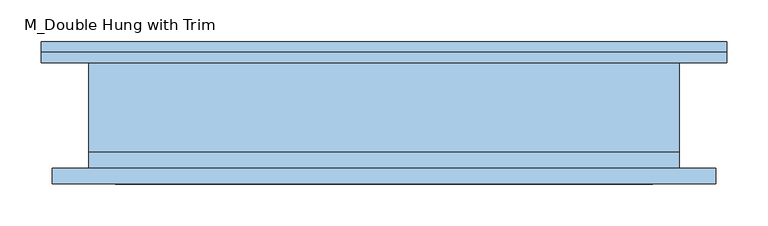
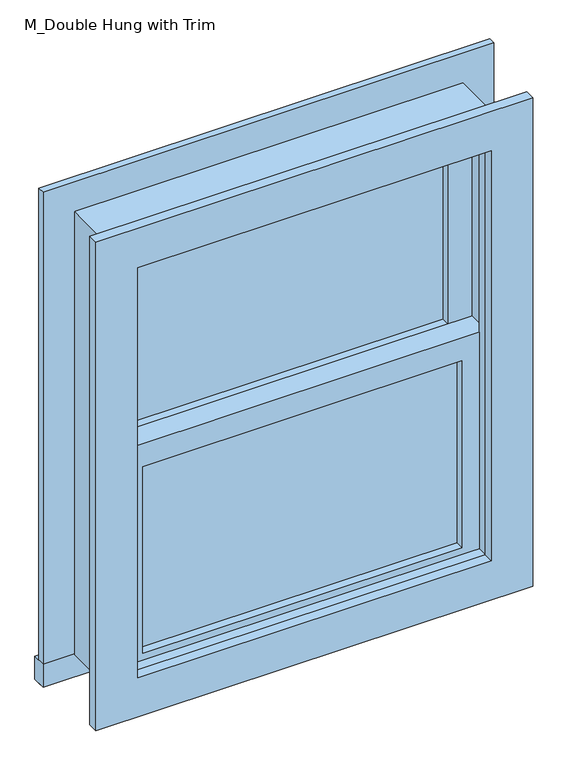
"""IFC4 building model written with IfcOpenShell, lengths in millimetres: window geometry, M_Double Hung with Trim."""

from ifc_helpers import new_model, si_unit, frame, origin, place, context, project, spatial, polyline, outline, extrude, source, transform, mapped, element, save


def m_double_hung_with_trim_a11a7e0a(model_context):
    return source(origin(), model_context, "Body", "SweptSolid", [
        extrude(outline(polyline([(-292.1, -15.825), (292.1, -15.825), (292.1, -28.525), (-292.1, -28.525), (-292.1, -15.825)])), frame((0.0, 0.0, 628.65), z_axis=(0.0, 0.0, 1.0), x_axis=(1.0, 0.0, 0.0)), (0.0, 0.0, 1.0), 361.95),
        extrude(outline(polyline([(1035.05, -336.55), (584.2, -336.55), (584.2, 336.55), (1035.05, 336.55), (1035.05, -336.55)]), holes=[polyline([(990.6, -292.1), (990.6, 292.1), (628.65, 292.1), (628.65, -292.1), (990.6, -292.1)])]), frame((0.0, -44.4, 0.0), z_axis=(0.0, 1.0, 0.0), x_axis=(0.0, 0.0, 1.0)), (0.0, 0.0, 1.0), 44.45),
        extrude(outline(polyline([(-412.75, 89.2), (412.75, 89.2), (412.75, 63.5), (-412.75, 63.5), (-412.75, 89.2)])), frame((0.0, 0.0, 539.75), z_axis=(0.0, 0.0, 1.0), x_axis=(1.0, 0.0, 0.0)), (0.0, 0.0, 1.0), 44.45),
        extrude(outline(polyline([(1498.6, -412.75), (539.75, -412.75), (539.75, 412.75), (1498.6, 412.75), (1498.6, -412.75)]), holes=[polyline([(1422.4, -336.55), (1422.4, 336.55), (584.2, 336.55), (584.2, -336.55), (1422.4, -336.55)])]), frame((0.0, 63.5, 0.0), z_axis=(0.0, 1.0, 0.0), x_axis=(0.0, 0.0, 1.0)), (0.0, 0.0, 1.0), 13.0),
        extrude(outline(polyline([(1485.9, 400.05), (1485.9, -400.05), (539.75, -400.05), (539.75, 400.05), (1485.9, 400.05)]), holes=[polyline([(1409.7, 323.85), (615.95, 323.85), (615.95, -323.85), (1409.7, -323.85), (1409.7, 323.85)])]), frame((0.0, -82.5, 0.0), z_axis=(0.0, 1.0, 0.0), x_axis=(0.0, 0.0, 1.0)), (0.0, 0.0, 1.0), 19.0),
        extrude(outline(polyline([(292.1, 15.925), (-292.1, 15.925), (-292.1, 28.625), (292.1, 28.625), (292.1, 15.925)])), frame((0.0, 0.0, 1035.05), z_axis=(0.0, 0.0, 1.0), x_axis=(1.0, 0.0, 0.0)), (0.0, 0.0, 1.0), 342.9),
        extrude(outline(polyline([(1422.4, -336.55), (990.6, -336.55), (990.6, 336.55), (1422.4, 336.55), (1422.4, -336.55)]), holes=[polyline([(1377.95, -292.1), (1377.95, 292.1), (1035.05, 292.1), (1035.05, -292.1), (1377.95, -292.1)])]), frame((0.0, 0.05, 0.0), z_axis=(0.0, 1.0, 0.0), x_axis=(0.0, 0.0, 1.0)), (0.0, 0.0, 1.0), 44.45),
        extrude(outline(polyline([(1441.45, -355.6), (584.2, -355.6), (584.2, 355.6), (1441.45, 355.6), (1441.45, -355.6)]), holes=[polyline([(1409.7, -323.85), (1409.7, 323.85), (615.95, 323.85), (615.95, -323.85), (1409.7, -323.85)])]), frame((0.0, -63.5, 0.0), z_axis=(0.0, 1.0, 0.0), x_axis=(0.0, 0.0, 1.0)), (0.0, 0.0, 1.0), 19.1),
        extrude(outline(polyline([(1441.45, 355.6), (1441.45, -355.6), (584.2, -355.6), (584.2, 355.6), (1441.45, 355.6)]), holes=[polyline([(1422.4, 336.55), (603.25, 336.55), (603.25, -336.55), (1422.4, -336.55), (1422.4, 336.55)])]), frame((0.0, -44.4, 0.0), z_axis=(0.0, 1.0, 0.0), x_axis=(0.0, 0.0, 1.0)), (0.0, 0.0, 1.0), 107.9),
    ])


if __name__ == "__main__":
    model = new_model("IFC4")
    model_context = context("Model", 3, world=origin())
    ifc_project = project(units=[si_unit("LENGTHUNIT", "METRE", prefix="MILLI")], contexts=[model_context])
    site = spatial("IfcSite", under=ifc_project)
    building = spatial("IfcBuilding", under=site)
    placement = place(None, origin())
    m_double_hung_with_trim_shape = m_double_hung_with_trim_a11a7e0a(model_context)
    element("IfcWindow", 1, ObjectType="M_Double Hung with Trim : 2'  4\" x 2'  9 3/4\"", at=placement, inside=building, context=model_context, shape_type="MappedRepresentation", body=[
        mapped(m_double_hung_with_trim_shape, transform((0.0, 0.0, 0.0), x_axis=(1.0, 0.0, 0.0), y_axis=(0.0, 1.0, 0.0), z_axis=(0.0, 0.0, 1.0))),
    ])
    save(model, "model.ifc")

# Revit data of these elements
# Type "M_Double Hung with Trim : 2'  4\" x 2'  9 3/4\""
#   Type Mark = "67"
#   Construction Type Id = "GSP4R"
#   Analytic Construction = "1/8 in Pilkington single glazing"
#   Visual Light Transmittance = 0.9
#   Thermal Resistance (R) = 0.271106 (m²·K)/W
#   Solar Heat Gain Coefficient = 0.78
#   Heat Transfer Coefficient (U) = 3.6886 W/(m²·K)
#   Height = 2' - 9 3/4"
#   Default Sill Height = 1' - 11"
#   Trim Projection - Ext. = 0' - 0.51181"
#   Trim Projection - Int. = 0' - 0.74803"
#   Trim Width - Exterior = 0' - 3"
#   Trim Width - Interior = 0' - 3"
#   Width = 2' - 4"
#   Window Inset = 0' - 0.74803"
#   Glass Pane Material = EXISTING WINDOW
#   Sash = Trim
#   Trim Exterior Material = Trim
#   Trim Interior Material = Trim
#   Wall Closure = (empty or 0)
# Element 1 (IfcWindow, "M_Double Hung with Trim : 2'  4\" x 2'  9 3/4\"")
#   Materials on its faces: "Trim", "EXISTING WINDOW"
# Materials
#   "EXISTING WINDOW": class "Glass", colour RGB 218 227 224, transparency 0.85, Description = "Soda Lime Glass", Cost = 0
#   "Trim": class "Wood", colour RGB 250 251 245, transparency 0, Cost = 0
